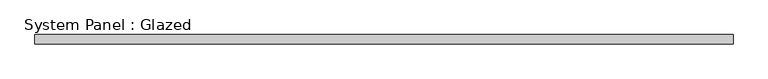
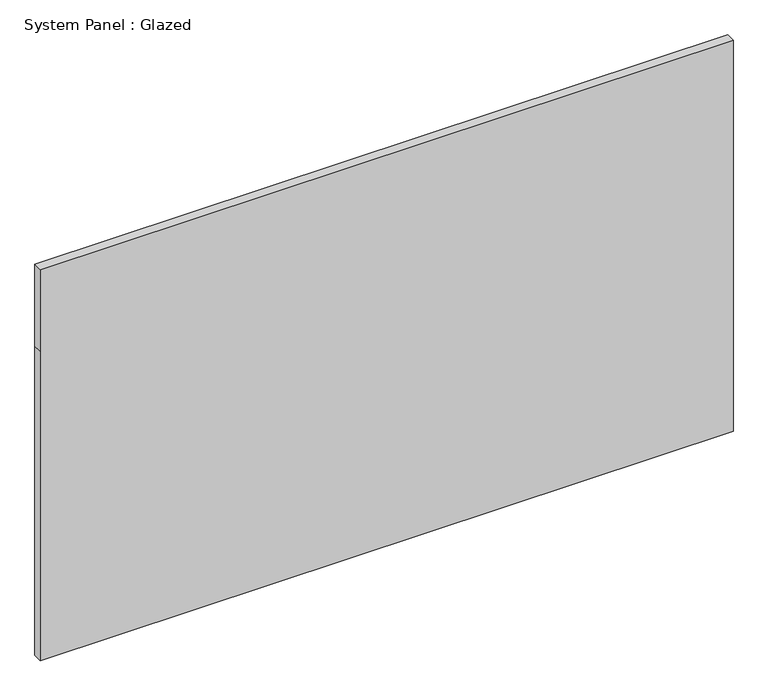
"""IFC4 building model written with IfcOpenShell, lengths in millimetres: plate geometry, System Panel : Glazed."""

from ifc_helpers import new_model, si_unit, frame, origin, place, context, project, spatial, polyline, outline, extrude, source, transform, mapped, element, save


def system_panel_glazed_d60e1f89(model_context):
    return source(origin(), model_context, "Body", "SweptSolid", [
        extrude(outline(polyline([(0.0, -968.375), (0.0, 968.375), (914.4, 968.375), (1155.7, 968.375), (1155.7, -968.375), (914.4, -968.375), (0.0, -968.375)])), frame((0.0, 19.05, 0.0), z_axis=(0.0, 1.0, 0.0), x_axis=(0.0, 0.0, 1.0)), (0.0, 0.0, 1.0), 25.4),
    ])


if __name__ == "__main__":
    model = new_model("IFC4")
    model_context = context("Model", 3, world=origin())
    ifc_project = project(units=[si_unit("LENGTHUNIT", "METRE", prefix="MILLI")], contexts=[model_context])
    site = spatial("IfcSite", under=ifc_project)
    building = spatial("IfcBuilding", under=site)
    placement = place(None, origin())
    system_panel_glazed_shape = system_panel_glazed_d60e1f89(model_context)
    element("IfcPlate", 1, ObjectType="System Panel : Glazed", at=placement, inside=building, context=model_context, shape_type="MappedRepresentation", body=[
        mapped(system_panel_glazed_shape, transform((0.0, 0.0, 0.0), x_axis=(1.0, 0.0, 0.0), y_axis=(0.0, 1.0, 0.0), z_axis=(0.0, 0.0, 1.0))),
    ])
    save(model, "model.ifc")

# Revit data of these elements
# Element 1 (IfcPlate, "System Panel : Glazed")
#   Materials on its faces: "Glass"
# Materials
#   "Glass": class "Glass", colour RGB 0 128 192, transparency 0.75, Cost = 0
